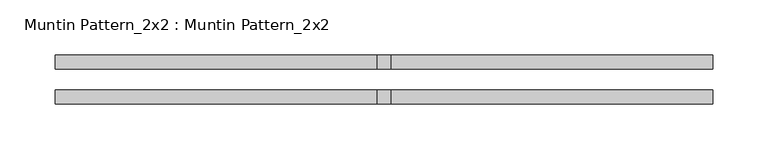
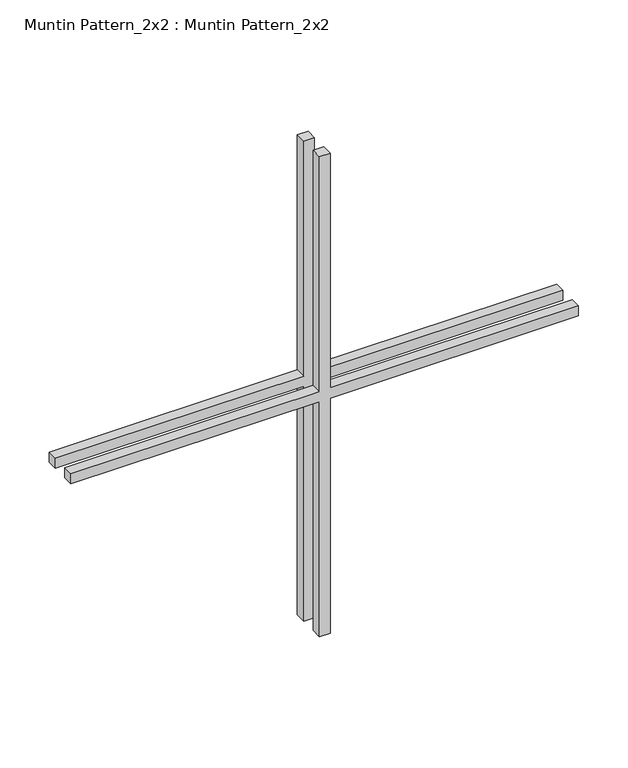
"""IFC4 building model written with IfcOpenShell, lengths in millimetres: proxy geometry, Muntin Pattern_2x2 : Muntin Pattern_2x2."""

from ifc_helpers import new_model, si_unit, frame, origin, place, context, project, spatial, polyline, outline, extrude, source, transform, mapped, element, save


def muntin_pattern_2x2_muntin_pattern_2x2_c5be7895(model_context):
    return source(origin(), model_context, "Body", "SweptSolid", [
        extrude(outline(polyline([(304.8, -6.35), (304.8, -298.45), (292.1, -298.45), (292.1, -6.35), (0.0, -6.35), (0.0, 6.35), (292.1, 6.35), (292.1, 298.45), (304.8, 298.45), (304.8, 6.35), (596.9, 6.35), (596.9, -6.35), (304.8, -6.35)])), frame((0.0, 9.525, 0.0), z_axis=(0.0, 1.0, 0.0), x_axis=(0.0, 0.0, 1.0)), (0.0, 0.0, 1.0), 12.7),
        extrude(outline(polyline([(304.8, -6.35), (304.8, -298.45), (292.1, -298.45), (292.1, -6.35), (0.0, -6.35), (0.0, 6.35), (292.1, 6.35), (292.1, 298.45), (304.8, 298.45), (304.8, 6.35), (596.9, 6.35), (596.9, -6.35), (304.8, -6.35)])), frame((0.0, -22.225, 0.0), z_axis=(0.0, 1.0, 0.0), x_axis=(0.0, 0.0, 1.0)), (0.0, 0.0, 1.0), 12.7),
    ])


if __name__ == "__main__":
    model = new_model("IFC4")
    model_context = context("Model", 3, world=origin())
    ifc_project = project(units=[si_unit("LENGTHUNIT", "METRE", prefix="MILLI")], contexts=[model_context])
    site = spatial("IfcSite", under=ifc_project)
    building = spatial("IfcBuilding", under=site)
    placement = place(None, origin())
    muntin_pattern_2x2_muntin_pattern_2x2_shape = muntin_pattern_2x2_muntin_pattern_2x2_c5be7895(model_context)
    element("IfcBuildingElementProxy", 1, Name="Muntin Pattern_2x2 : Muntin Pattern_2x2", ObjectType="Muntin Pattern_2x2 : Muntin Pattern_2x2", at=placement, inside=building, context=model_context, shape_type="MappedRepresentation", body=[
        mapped(muntin_pattern_2x2_muntin_pattern_2x2_shape, transform((0.0, 0.0, 0.0), x_axis=(1.0, 0.0, 0.0), y_axis=(0.0, 1.0, 0.0), z_axis=(0.0, 0.0, 1.0))),
    ])
    save(model, "model.ifc")

# Revit data of these elements
# Type "Muntin Pattern_2x2 : Muntin Pattern_2x2"
#   Width [instance default] = 4' - 0"
#   Thickness = 0' - 0 1/2"
#   Height [instance default] = 4' - 0"
#   Distance = 0' - 0 3/4"
#   Interior Material [instance default] = none
#   Exterior Material [instance default] = none
# Element 1 (IfcBuildingElementProxy, "Muntin Pattern_2x2 : Muntin Pattern_2x2")
#   Width = 1' - 11 1/2"
#   Height = 1' - 11 1/2"
#   Interior Material = Wood - Stained
#   Exterior Material = Clad - White
#   Materials on its faces: "Clad - White", "Wood - Stained"
# Materials
#   "Clad - White": class "Wood", colour RGB 242 242 238, transparency 0, Cost = 0
#   "Wood - Stained": class "Wood", colour RGB 224 178 126, transparency 0, Cost = 0
